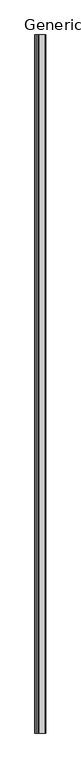
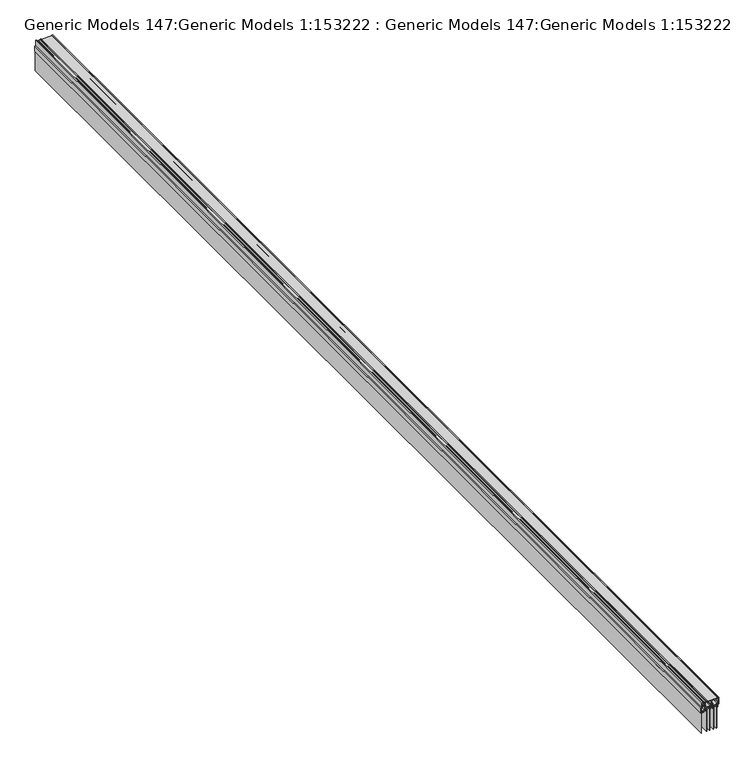
"""IFC4 building model written with IfcOpenShell, lengths in millimetres: proxy geometry, Generic Models 147:Generic Models 1:153222 : Generic Models 147:Generic Models 1:153222."""

from ifc_helpers import new_model, si_unit, frame, origin, place, context, project, spatial, polyline, outline, extrude, source, transform, mapped, element, save


def generic_models_147_generic_models_1_153222_generic_models_8b9d6566(model_context):
    return source(origin(), model_context, "Body", "SweptSolid", [
        extrude(outline(polyline([(-6572.0516395, -5303.1974793), (-6572.0516395, 2583.5025207), (-6557.721808, 2583.5025207), (-6557.721808, -5303.1974793), (-6572.0516395, -5303.1974793)])), frame((0.0, 0.0, 2827.2245908), z_axis=(0.0, 0.0, 1.0), x_axis=(1.0, 0.0, 0.0)), (0.0, 0.0, 1.0), 7.9798298),
        extrude(outline(polyline([(-6556.928058, -5303.1974793), (-6556.928058, 2583.5025207), (-6552.1867238, 2583.5025207), (-6552.1867238, -5303.1974793), (-6556.928058, -5303.1974793)])), frame((0.0, 0.0, 2668.0725763), z_axis=(0.0, 0.0, 1.0), x_axis=(1.0, 0.0, 0.0)), (0.0, 0.0, 1.0), 167.9255943),
        extrude(outline(polyline([(-6577.5867238, -5303.1974793), (-6577.5867238, 2583.5025207), (-6572.8453895, 2583.5025207), (-6572.8453895, -5303.1974793), (-6577.5867238, -5303.1974793)])), frame((0.0, 0.0, 2668.0725763), z_axis=(0.0, 0.0, 1.0), x_axis=(1.0, 0.0, 0.0)), (0.0, 0.0, 1.0), 167.9255943),
        extrude(outline(polyline([(2855.6408356, -6550.0700563), (2842.348162, -6550.0700563), (2842.348162, -6579.7033905), (2855.6408356, -6579.7033905), (2855.6408356, -6582.0740571), (2818.472169, -6582.0740571), (2818.472169, -6579.1953905), (2839.8928356, -6579.1953905), (2839.8928356, -6550.0700571), (2818.472169, -6550.0700571), (2818.472169, -6547.6993905), (2855.6408356, -6547.6993905), (2855.6408356, -6550.0700563)])), frame((0.0, -5303.1974793, 0.0), z_axis=(0.0, 1.0, 0.0), x_axis=(0.0, 0.0, 1.0)), (0.0, 0.0, 1.0), 7886.7),
        extrude(outline(polyline([(-6620.3963019, -5303.1974793), (-6620.3963019, 2583.5025207), (-6606.0664704, 2583.5025207), (-6606.0664704, -5303.1974793), (-6620.3963019, -5303.1974793)])), frame((0.0, 0.0, 2827.2245908), z_axis=(0.0, 0.0, 1.0), x_axis=(1.0, 0.0, 0.0)), (0.0, 0.0, 1.0), 7.9798298),
        extrude(outline(polyline([(-6605.2727204, -5303.1974793), (-6605.2727204, 2583.5025207), (-6600.5313862, 2583.5025207), (-6600.5313862, -5303.1974793), (-6605.2727204, -5303.1974793)])), frame((0.0, 0.0, 2668.0725763), z_axis=(0.0, 0.0, 1.0), x_axis=(1.0, 0.0, 0.0)), (0.0, 0.0, 1.0), 167.9255943),
        extrude(outline(polyline([(-6625.9313862, -5303.1974793), (-6625.9313862, 2583.5025207), (-6621.1900519, 2583.5025207), (-6621.1900519, -5303.1974793), (-6625.9313862, -5303.1974793)])), frame((0.0, 0.0, 2668.0725763), z_axis=(0.0, 0.0, 1.0), x_axis=(1.0, 0.0, 0.0)), (0.0, 0.0, 1.0), 167.9255943),
        extrude(outline(polyline([(2855.6408356, -6598.4147187), (2842.348162, -6598.4147187), (2842.348162, -6628.0480529), (2855.6408356, -6628.0480529), (2855.6408356, -6630.4187196), (2818.472169, -6630.4187196), (2818.472169, -6627.5400529), (2839.8928356, -6627.5400529), (2839.8928356, -6598.4147196), (2818.472169, -6598.4147196), (2818.472169, -6596.0440529), (2855.6408356, -6596.0440529), (2855.6408356, -6598.4147187)])), frame((0.0, -5303.1974793, 0.0), z_axis=(0.0, 1.0, 0.0), x_axis=(0.0, 0.0, 1.0)), (0.0, 0.0, 1.0), 7886.7),
        extrude(outline(polyline([(2876.6125066, -6561.956065), (2877.4001629, -6561.1613724), (2878.4161551, -6560.5687221), (2878.4161551, -6545.2440554), (2878.2468218, -6544.3127221), (2877.6541551, -6543.5507221), (2876.8921551, -6542.9580554), (2875.9608218, -6542.7887221), (2848.8674927, -6542.6193716), (2848.8674927, -6544.2280399), (2838.1148346, -6544.2280399), (2838.1148346, -6540.0793716), (2885.8668235, -6540.0793716), (2885.8668235, -6546.4293732), (2884.2581568, -6546.4293732), (2884.2581568, -6541.8342823), (2882.7341568, -6542.1113732), (2881.8874901, -6542.7040399), (2881.3794901, -6543.4660399), (2881.2101706, -6544.3972972), (2881.2101706, -6623.8993913), (2884.258162, -6623.8993913), (2884.258162, -6619.412058), (2885.8668287, -6619.412058), (2885.8668287, -6625.762058), (2881.1254954, -6625.762058), (2880.2788287, -6652.432058), (2884.258162, -6652.432058), (2884.258162, -6648.0293913), (2885.8668287, -6648.0293913), (2885.8668287, -6654.3793913), (2852.5081568, -6654.3793913), (2852.5081568, -6652.4320563), (2878.416168, -6652.4320563), (2878.416168, -6637.6153766), (2878.2468346, -6636.6840433), (2877.654168, -6635.9220433), (2876.892168, -6635.4140433), (2875.9608346, -6635.1600433), (2838.1148346, -6635.1600433), (2838.1148346, -6631.3500477), (2847.8797119, -6631.3500477), (2848.867491, -6632.6200494), (2875.9608296, -6632.450716), (2876.8921629, -6632.2813827), (2877.6541629, -6631.688716), (2878.2468296, -6630.926716), (2878.4161629, -6629.9953827), (2878.4161629, -6617.5493827), (2877.4001629, -6616.956716), (2876.621304, -6616.127702), (2876.0561457, -6615.215427), (2875.7091033, -6614.2484162), (2875.5845921, -6613.2551952), (2875.6870271, -6612.2642893), (2876.0208238, -6611.3042238), (2876.588876, -6610.4020029), (2877.4001629, -6609.590716), (2878.4161698, -6608.9133879), (2878.4161698, -6590.0327152), (2848.8674927, -6590.0327152), (2848.8674927, -6591.895381), (2838.1148346, -6591.895381), (2838.1148346, -6585.5453732), (2848.867491, -6585.5453732), (2848.867491, -6587.4080391), (2878.4161629, -6587.2233599), (2878.4161629, -6569.1200391), (2877.4021183, -6568.525417), (2876.6093812, -6567.7326798), (2876.0454301, -6566.829938), (2875.7078631, -6565.8551634), (2875.5962337, -6564.8443724), (2875.7100955, -6563.8335814), (2876.0490019, -6562.8588068), (2876.6125066, -6561.956065)])), frame((0.0, -5303.1974793, 0.0), z_axis=(0.0, 1.0, 0.0), x_axis=(0.0, 0.0, 1.0)), (0.0, 0.0, 1.0), 7886.7),
        extrude(outline(polyline([(2809.6668373, -6660.8987177), (2809.6668373, -6659.3112177), (2668.0725763, -6659.3112177), (2668.0725763, -6658.5174677), (2809.6668373, -6658.5174677), (2809.6668373, -6640.1553785), (2815.8475013, -6640.1553785), (2815.8475013, -6637.1073732), (2868.6794945, -6637.1073732), (2868.6794945, -6638.3773776), (2855.7255048, -6638.3773776), (2855.7255048, -6649.5533776), (2868.6795048, -6649.5533776), (2868.6795048, -6650.8233913), (2848.5719542, -6650.8233913), (2846.0055975, -6660.8987177), (2809.6668373, -6660.8987177)]), holes=[polyline([(2854.455491, -6649.5533854), (2854.455491, -6638.4620382), (2826.8541723, -6638.4620382), (2826.8541723, -6648.6220494), (2825.2454954, -6648.6220494), (2825.2454954, -6638.3773862), (2817.1174927, -6638.3773862), (2817.1174927, -6641.4253913), (2810.9368304, -6641.4253913), (2810.9368304, -6652.3473879), (2817.117504, -6652.3473879), (2817.117504, -6659.544052), (2840.0621732, -6659.544052), (2840.0621732, -6657.1733854), (2841.3321543, -6657.1733854), (2841.3321543, -6659.544052), (2845.0792221, -6659.544052), (2847.5547856, -6649.5533854), (2854.455491, -6649.5533854)])]), frame((0.0, -5303.1974793, 0.0), z_axis=(0.0, 1.0, 0.0), x_axis=(0.0, 0.0, 1.0)), (0.0, 0.0, 1.0), 7886.7),
    ])


if __name__ == "__main__":
    model = new_model("IFC4")
    model_context = context("Model", 3, world=origin())
    ifc_project = project(units=[si_unit("LENGTHUNIT", "METRE", prefix="MILLI")], contexts=[model_context])
    site = spatial("IfcSite", under=ifc_project)
    building = spatial("IfcBuilding", under=site)
    placement = place(None, origin())
    generic_models_147_generic_models_1_153222_generic_models_shape = generic_models_147_generic_models_1_153222_generic_models_8b9d6566(model_context)
    element("IfcBuildingElementProxy", 1, Name="Generic Models 147:Generic Models 1:153222 : Generic Models 147:Generic Models 1:153222", ObjectType="Generic Models 147:Generic Models 1:153222 : Generic Models 147:Generic Models 1:153222", at=placement, inside=building, context=model_context, shape_type="MappedRepresentation", body=[
        mapped(generic_models_147_generic_models_1_153222_generic_models_shape, transform((0.0, 0.0, 0.0), x_axis=(1.0, 0.0, 0.0), y_axis=(0.0, 1.0, 0.0), z_axis=(0.0, 0.0, 1.0))),
    ])
    save(model, "model.ifc")

# Revit data of these elements
# Type "Generic Models 147:Generic Models 1:153222 : Generic Models 147:Generic Models 1:153222"
#   NameOverride = "Generic Models 147:Generic Models 1:153222"
#   ObjectTypeOverride = "Generic Models 147:Generic Models 1"
#   Reference = "Generic Models 1"
#   Category = "Generic Models"
#   Tag = "153222"
# Element 1 (IfcBuildingElementProxy, "Generic Models 147:Generic Models 1:153222 : Generic Models 147:Generic Models 1:153222")
#   Materials on its faces: "_SIDING DOOR PER SCHEDULE 11160"
# Materials
#   "_SIDING DOOR PER SCHEDULE 11160": class "Unassigned", colour RGB 255 255 255, transparency 0
